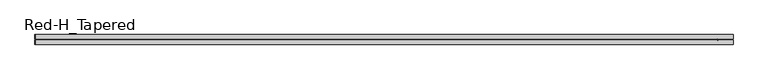
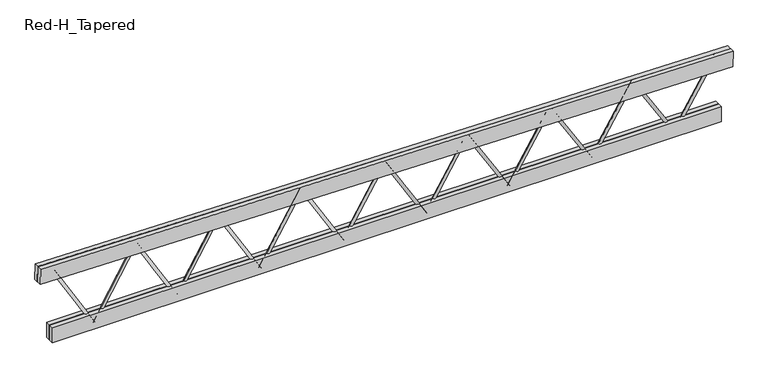
"""IFC4 building model written with IfcOpenShell, lengths in millimetres: beam geometry, Construction_Frames_RedBuilt_Openweb_Red-H_Tapered : Red-H_Tapered."""

from ifc_helpers import new_model, si_unit, point, frame, origin, origin_2d, place, context, project, spatial, polyline, circle_curve, trimmed, segment, composite_curve, outline, extrude, source, transform, mapped, element, save


def red_h_tapered_a0183158(model_context):
    return source(origin(), model_context, "Body", "SweptSolid", [
        extrude(outline(composite_curve([segment(trimmed(circle_curve(origin_2d(), 12.7), [point((0.0, 12.7))], [point((0.0, -12.7))], False, "CARTESIAN"), True, "CONTINUOUS"), segment(trimmed(circle_curve(origin_2d(), 12.7), [point((0.0, -12.7))], [point((0.0, 12.7))], False, "CARTESIAN"), True, "CONTINUOUS")], self_intersect=False)), frame((2516.6154336, 0.0, -367.0101562), z_axis=(0.5241067286958753, 0.0, 0.8516525916920046), x_axis=(0.0, -1.0, 0.0)), (0.0, 0.0, 1.0), 685.9604558),
        extrude(outline(composite_curve([segment(trimmed(circle_curve(origin_2d(), 12.7), [point((0.0, -12.7))], [point((0.0, 12.6999999))], False, "CARTESIAN"), True, "CONTINUOUS"), segment(trimmed(circle_curve(origin_2d(), 12.7), [point((0.0, 12.6999999))], [point((0.0, -12.7))], False, "CARTESIAN"), True, "CONTINUOUS")], self_intersect=False)), frame((2516.6154336, 0.0, -367.0101562), z_axis=(-0.5215353438102012, 0.0, 0.853229679017775), x_axis=(0.0, -1.0, 0.0)), (0.0, 0.0, 1.0), 689.3425245),
        extrude(outline(composite_curve([segment(trimmed(circle_curve(origin_2d(), 12.7), [point((0.0, 12.7))], [point((0.0, -12.6999999))], False, "CARTESIAN"), True, "CONTINUOUS"), segment(trimmed(circle_curve(origin_2d(), 12.7), [point((0.0, -12.6999999))], [point((0.0, 12.7))], False, "CARTESIAN"), True, "CONTINUOUS")], self_intersect=False)), frame((1797.5824526, 0.0, -367.0101562), z_axis=(0.5215353438102003, 0.0, 0.8532296790177755), x_axis=(0.0, -1.0, 0.0)), (0.0, 0.0, 1.0), 689.3425245),
        extrude(outline(composite_curve([segment(trimmed(circle_curve(origin_2d(), 12.7), [point((0.0, -12.7))], [point((0.0, 12.7))], False, "CARTESIAN"), True, "CONTINUOUS"), segment(trimmed(circle_curve(origin_2d(), 12.7), [point((0.0, 12.7))], [point((0.0, -12.7))], False, "CARTESIAN"), True, "CONTINUOUS")], self_intersect=False)), frame((1797.5824526, 0.0, -367.0101562), z_axis=(-0.5189844139237941, 0.0, 0.8547837025260694), x_axis=(0.0, -1.0, 0.0)), (0.0, 0.0, 1.0), 692.7308044),
        extrude(outline(composite_curve([segment(trimmed(circle_curve(origin_2d(), 12.7), [point((0.0, 12.7000001))], [point((0.0, -12.7))], False, "CARTESIAN"), True, "CONTINUOUS"), segment(trimmed(circle_curve(origin_2d(), 12.7), [point((0.0, -12.7))], [point((0.0, 12.7000001))], False, "CARTESIAN"), True, "CONTINUOUS")], self_intersect=False)), frame((1078.5494715, 0.0, -367.0101562), z_axis=(0.518984413923793, 0.0, 0.8547837025260702), x_axis=(0.0, -1.0, 0.0)), (0.0, 0.0, 1.0), 692.7308044),
        extrude(outline(composite_curve([segment(trimmed(circle_curve(origin_2d(), 12.7), [point((0.0, -12.7))], [point((0.0, 12.7))], False, "CARTESIAN"), True, "CONTINUOUS"), segment(trimmed(circle_curve(origin_2d(), 12.7), [point((0.0, 12.7))], [point((0.0, -12.7))], False, "CARTESIAN"), True, "CONTINUOUS")], self_intersect=False)), frame((1078.5494715, 0.0, -367.0101562), z_axis=(-0.5164537759218651, 0.0, 0.856315068964717), x_axis=(0.0, -1.0, 0.0)), (0.0, 0.0, 1.0), 696.1252048),
        extrude(outline(composite_curve([segment(trimmed(circle_curve(origin_2d(), 12.7), [point((0.0, 12.7))], [point((0.0, -12.7))], False, "CARTESIAN"), True, "CONTINUOUS"), segment(trimmed(circle_curve(origin_2d(), 12.7), [point((0.0, -12.7))], [point((0.0, 12.7))], False, "CARTESIAN"), True, "CONTINUOUS")], self_intersect=False)), frame((359.5164905, 0.0, -367.0101562), z_axis=(0.5164537759218657, 0.0, 0.8563150689647167), x_axis=(0.0, -1.0, 0.0)), (0.0, 0.0, 1.0), 696.1252048),
        extrude(outline(composite_curve([segment(trimmed(circle_curve(origin_2d(), 12.7), [point((0.0, -12.7))], [point((0.0, 12.7))], False, "CARTESIAN"), True, "CONTINUOUS"), segment(trimmed(circle_curve(origin_2d(), 12.7), [point((0.0, 12.7))], [point((0.0, -12.7))], False, "CARTESIAN"), True, "CONTINUOUS")], self_intersect=False)), frame((359.5164905, 0.0, -367.0101562), z_axis=(-0.5139432662956527, 0.0, 0.8578241772236056), x_axis=(0.0, -1.0, 0.0)), (0.0, 0.0, 1.0), 699.5256366),
        extrude(outline(composite_curve([segment(trimmed(circle_curve(origin_2d(), 12.7), [point((0.0, -12.7))], [point((0.0, 12.7))], False, "CARTESIAN"), True, "CONTINUOUS"), segment(trimmed(circle_curve(origin_2d(), 12.7), [point((0.0, 12.7))], [point((0.0, -12.7))], False, "CARTESIAN"), True, "CONTINUOUS")], self_intersect=False)), frame((-359.5164905, 0.0, -367.0101562), z_axis=(0.5139432662956213, 0.0, 0.8578241772236244), x_axis=(0.0, -1.0, 0.0)), (0.0, 0.0, 1.0), 699.5256366),
        extrude(outline(composite_curve([segment(trimmed(circle_curve(origin_2d(), 12.7), [point((0.0, 12.7))], [point((0.0, -12.7))], False, "CARTESIAN"), True, "CONTINUOUS"), segment(trimmed(circle_curve(origin_2d(), 12.7), [point((0.0, -12.7))], [point((0.0, 12.7))], False, "CARTESIAN"), True, "CONTINUOUS")], self_intersect=False)), frame((-359.5164905, 0.0, -367.0101562), z_axis=(-0.511452721242837, 0.0, 0.8593114184818545), x_axis=(0.0, -1.0, 0.0)), (0.0, 0.0, 1.0), 702.9320123),
        extrude(outline(composite_curve([segment(trimmed(circle_curve(origin_2d(), 12.7), [point((0.0, -12.7))], [point((0.0, 12.7))], False, "CARTESIAN"), True, "CONTINUOUS"), segment(trimmed(circle_curve(origin_2d(), 12.7), [point((0.0, 12.7))], [point((0.0, -12.7))], False, "CARTESIAN"), True, "CONTINUOUS")], self_intersect=False)), frame((-1078.5494715, 0.0, -367.0101562), z_axis=(0.5114527212428354, 0.0, 0.8593114184818554), x_axis=(0.0, -1.0, 0.0)), (0.0, 0.0, 1.0), 702.9320123),
        extrude(outline(composite_curve([segment(trimmed(circle_curve(origin_2d(), 12.7), [point((0.0, 12.7))], [point((0.0, -12.7000001))], False, "CARTESIAN"), True, "CONTINUOUS"), segment(trimmed(circle_curve(origin_2d(), 12.7), [point((0.0, -12.7000001))], [point((0.0, 12.7))], False, "CARTESIAN"), True, "CONTINUOUS")], self_intersect=False)), frame((-1078.5494715, 0.0, -367.0101562), z_axis=(-0.5089819767631879, 0.0, 0.8607771763529966), x_axis=(0.0, -1.0, 0.0)), (0.0, 0.0, 1.0), 706.3442458),
        extrude(outline(composite_curve([segment(trimmed(circle_curve(origin_2d(), 12.7), [point((0.0, -12.7))], [point((0.0, 12.7000001))], False, "CARTESIAN"), True, "CONTINUOUS"), segment(trimmed(circle_curve(origin_2d(), 12.7), [point((0.0, 12.7000001))], [point((0.0, -12.7))], False, "CARTESIAN"), True, "CONTINUOUS")], self_intersect=False)), frame((-1797.5824526, 0.0, -367.0101562), z_axis=(0.508981976763201, 0.0, 0.8607771763529889), x_axis=(0.0, -1.0, 0.0)), (0.0, 0.0, 1.0), 706.3442458),
        extrude(outline(composite_curve([segment(trimmed(circle_curve(origin_2d(), 12.7), [point((0.0, 12.7))], [point((0.0, -12.7))], False, "CARTESIAN"), True, "CONTINUOUS"), segment(trimmed(circle_curve(origin_2d(), 12.7), [point((0.0, -12.7))], [point((0.0, 12.7))], False, "CARTESIAN"), True, "CONTINUOUS")], self_intersect=False)), frame((-1797.5824526, 0.0, -367.0101562), z_axis=(-0.5065308687490784, 0.0, 0.8622218270284648), x_axis=(0.0, -1.0, 0.0)), (0.0, 0.0, 1.0), 709.7622528),
        extrude(outline(composite_curve([segment(trimmed(circle_curve(origin_2d(), 12.7), [point((0.0, -12.7))], [point((0.0, 12.7))], False, "CARTESIAN"), True, "CONTINUOUS"), segment(trimmed(circle_curve(origin_2d(), 12.7), [point((0.0, 12.7))], [point((0.0, -12.7))], False, "CARTESIAN"), True, "CONTINUOUS")], self_intersect=False)), frame((-2516.6154336, 0.0, -367.0101562), z_axis=(0.5065308687490667, 0.0, 0.8622218270284718), x_axis=(0.0, -1.0, 0.0)), (0.0, 0.0, 1.0), 709.7622528),
        extrude(outline(composite_curve([segment(trimmed(circle_curve(origin_2d(), 12.7), [point((0.0, 12.7))], [point((0.0, -12.7))], False, "CARTESIAN"), True, "CONTINUOUS"), segment(trimmed(circle_curve(origin_2d(), 12.7), [point((0.0, -12.7))], [point((0.0, 12.7))], False, "CARTESIAN"), True, "CONTINUOUS")], self_intersect=False)), frame((-2516.6154336, 0.0, -367.0101562), z_axis=(-0.5040992330715739, 0.0, 0.8636457394190346), x_axis=(0.0, -1.0, 0.0)), (0.0, 0.0, 1.0), 713.1859502),
        extrude(outline(polyline([(-2901.5319241, -41.275), (-2901.5319241, -3.175), (2901.5319241, -3.175), (2901.5319241, -41.275), (-2901.5319241, -41.275)])), frame((0.0, 0.0, -386.0601562), z_axis=(0.0, 0.0, 1.0), x_axis=(1.0, 0.0, 0.0)), (0.0, 0.0, 1.0), 139.7),
        extrude(outline(polyline([(-2901.5319241, 3.175), (-2901.5319241, 41.275), (2901.5319241, 41.275), (2901.5319241, 3.175), (-2901.5319241, 3.175)])), frame((0.0, 0.0, -386.0601562), z_axis=(0.0, 0.0, 1.0), x_axis=(1.0, 0.0, 0.0)), (0.0, 0.0, 1.0), 139.7),
        extrude(outline(polyline([(0.0, -38.1), (0.0, 0.0), (6007.123103, 0.0), (6007.123103, -38.1), (0.0, -38.1)])), frame((-3005.4947057, -3.175, 185.4598263), z_axis=(0.01691325419131241, 0.0, 0.9998569606862074), x_axis=(0.9998569606862074, 0.0, -0.01691325419131241)), (0.0, 0.0, 1.0), 139.7),
        extrude(outline(polyline([(0.0, -38.1), (0.0, 0.0), (6007.123103, 0.0), (6007.123103, -38.1), (0.0, -38.1)])), frame((-3005.4947057, 41.275, 185.4598263), z_axis=(0.01691325419131241, 0.0, 0.9998569606862074), x_axis=(0.9998569606862074, 0.0, -0.01691325419131241)), (0.0, 0.0, 1.0), 139.7),
    ])


if __name__ == "__main__":
    model = new_model("IFC4")
    model_context = context("Model", 3, world=origin())
    ifc_project = project(units=[si_unit("LENGTHUNIT", "METRE", prefix="MILLI")], contexts=[model_context])
    site = spatial("IfcSite", under=ifc_project)
    building = spatial("IfcBuilding", under=site)
    placement = place(None, origin())
    red_h_tapered_shape = red_h_tapered_a0183158(model_context)
    element("IfcBeam", 1, ObjectType="Construction_Frames_RedBuilt_Openweb_Red-H_Tapered : Red-H_Tapered", at=placement, inside=building, context=model_context, shape_type="MappedRepresentation", body=[
        mapped(red_h_tapered_shape, transform((0.0, 0.0, 0.0), x_axis=(1.0, 0.0, 0.0), y_axis=(0.0, 1.0, 0.0), z_axis=(0.0, 0.0, 1.0))),
    ])
    save(model, "model.ifc")

# Revit data of these elements
# Type "Construction_Frames_RedBuilt_Openweb_Red-H_Tapered : Red-H_Tapered"
#   Youtube clip = ""
#   Weight Net (Kg) = "0"
#   Webs = "Up to 2\" diameter tubular steel"
#   Uniformat II Description = ""
#   Uniformat II Code = ""
#   Uniclass 2015 Name = "Softwood trusses"
#   Uniclass 2015 Code = "Pr_20_85_90_81"
#   Uniclass 2.0 Description = "Structural Framing Systems"
#   Uniclass 2.0 Code = "SS-15-10-75"
#   Uniclass 1.4 Description = "Trusses"
#   Uniclass 1.4 Code = "L3523"
#   UNSPSC Code = "30103606"
#   Technical description = "http://www.redbuilt.com/reference/literature-and-other-resources"
#   Region South America = "None"
#   Region Oceania = "None"
#   Region North America = "US"
#   Region Middle East = "None"
#   Region Europe = "None"
#   Region Asia = "None"
#   Region Antarctica = "None"
#   Region Africa = "None"
#   QR code = "http://bimobject.com/redbuilt/product/redbuilt-0003"
#   Product url = "http://www.redbuilt.com/products/default.aspx?id=2"
#   Product group = "Wood Trusses"
#   Product family = "Construction"
#   Product data url = "https://bimobject.com/redbuilt/product/redbuilt-0003"
#   Product certification = ""
#   Product SKU = "redbuilt-0003"
#   Product Page URL = "http://www.redbuilt.com/commercial-systems/red-m-red-h-open-web-trusses"
#   Product Guid = "2c5793f2-6ffb-4665-b825-cf90c048e711"
#   Product Documentation Link = "http://www.redbuilt.com/documents/OW_Guide_2017_07_LowRes_wLinks.pdf"
#   OmniClass Description = "Wood Trusses"
#   OmniClass Code = "23-13 35 19 13 17"
#   NBS Reference Description = ""
#   NBS Reference Code = ""
#   Material secondary = "Steel"
#   Material main = "CHARRED WOOD"
#   Masterformat 2014 Description = "Metal-Web Wood Joists"
#   Masterformat 2014 Code = "06 17 36"
#   Manufacturer name = "RedBuilt"
#   Manufacturer country = "United States"
#   Installation instructions = "http://www.redbuilt.com/documents/Installation_Sheets_Open-Web.pdf"
#   IFC Classification = ""
#   EAN code = ""
#   Design country = "United States"
#   Product Information = "http://redbuilt.com/products/default.aspx?id=2"
#   Model = "Red-H-Tapered"
#   Manufacturer URL = "http://redbuilt.com/"
#   Manufacturer = "RedBuilt™"
#   Description = "Open Web Truss"
#   Date of publishing = "8/17/2010"
#   Contact us = "http://redbuilt.com/contact/"
#   Chords = "Double 1½\" x 5½\" MSR lumber"
#   COBIe Type Category = ""
#   Brand url = "http://www.redbuilt.com"
#   BIMobject main category code = "construction"
#   BIMobject main category = "Construction"
#   BIMobject category code = "construction-frames-trusses"
#   BIMobject category = "Frames & Trusses"
#   Web Radius = 0' - 0 1/2"
#   Web Layout Offset Start [instance default] = 0' - 5"
#   Web Layout Offset End [instance default] = 0' - 5"
#   Web Diameter = 0' - 1"
#   TotalLength [instance default] = 20' - 0"
#   Span Minimum = 4' - 0"
#   Span Maximum = 70' - 0"
#   Span Limit [instance default] = 20' - 0"
#   Nominal width = 0' - 0"
#   Nominal height = 0' - 0"
#   Inner Depth Top [instance default] = 0' - 2.76372"
#   Depth Start [instance default] = 6' - 0"
#   Top Chord Length [instance default] = 20' - 1.19701"
#   TC Extension Start Aux [instance default] = 0' - 0"
#   TC Extension End Aux [instance default] = 0' - 0"
#   T-B Chord Length Difference L [instance default] = 0' - 4"
#   T-B Chord Length Difference [instance default] = 0' - 4"
#   Height 2 [instance default] = 6' - 0"
#   Depth Minimum at Wall = 2' - 0"
#   Depth Maximum at Wall = 6' - 0"
#   Depth Lower End [instance default] = 2' - 0"
#   Depth Higher End [instance default] = 6' - 0"
#   Depth End [instance default] = 2' - 0"
#   Depth 2 [instance default] = 2' - 0"
#   Chord Width = 0' - 3 1/4"
#   Chord Thickness = 0' - 1 1/2"
#   Chord Depth = 0' - 5 1/2"
#   Offset Start [instance default] = 0' - 0"
#   TC Extension Start [instance default] = 0' - 0"
#   End Panel = 0' - 5"
#   Offset End [instance default] = 0' - 0"
#   TC Extension End [instance default] = 0' - 0"
#   Length [instance default] = 20' - 0"
#   Angle [instance default] = 5.71059°
#   Span Limit Warning [instance default] = no
#   Edition number = 1
#   Top Bearing Start [instance default] = yes
#   Top Bearing End [instance default] = yes
#   Bottom Bearing Start [instance default] = no
#   Bottom Bearing End [instance default] = no
#   8 Panels [instance default] = yes
#   16 Panels [instance default] = no
#   12 Panels [instance default] = no
#   Web Material = RedBuilt-Steel, Galvanized
#   Clip Material = RedBuilt-Steel, Galvanized
#   Chords Material = WOOD-OAKFIRE
#   URL = ""
#   Assembly Code = ""
# Element 1 (IfcBeam, "Construction_Frames_RedBuilt_Openweb_Red-H_Tapered : Red-H_Tapered")
#   TotalLength = 19' - 8.46708"
#   Span Limit = 19' - 8.46708"
#   Inner Depth Top = 0' - 2.75039"
#   Depth Start = 5' - 0"
#   Top Chord Length = 19' - 8.50091"
#   Height 2 = 5' - 0"
#   Depth Higher End = 5' - 0"
#   Depth 2 = 0' - 4"
#   Angle = 0.969104°
#   Materials on its faces: "RedBuilt-Steel, Galvanized", "WOOD-OAKFIRE"
# Materials
#   "RedBuilt-Steel, Galvanized": class "Metal", colour RGB 164 172 176, transparency 0, Manufacturer = "RedBuilt. LLC", Comments = "Openweb Metal Web", URL = "http://www.redbuilt.com/", Description = "Galvanized steel", Cost = 0
#   "WOOD-OAKFIRE": class "Wood", colour RGB 198 202 183, transparency 0, Description = "Generic wood", Cost = 0
